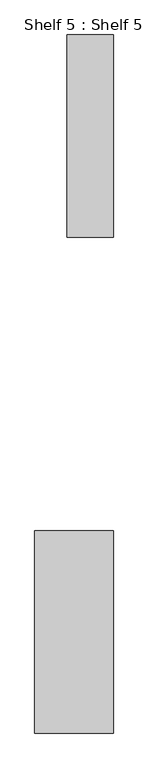
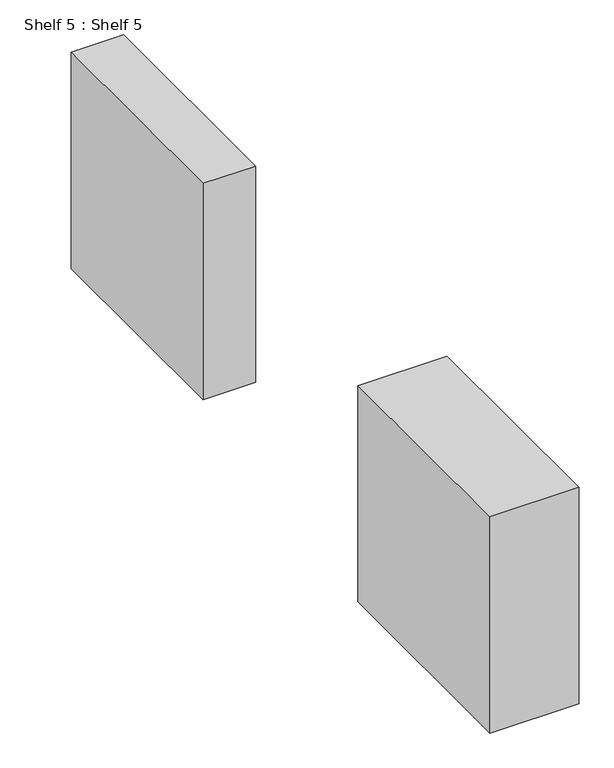
"""IFC4 building model written with IfcOpenShell, lengths in millimetres: furniture geometry, Shelf 5 : Shelf 5."""

from ifc_helpers import new_model, si_unit, origin, origin_with_axes, place, context, project, spatial, polyline, outline, extrude, source, transform, mapped, element, save


def shelf_5_shelf_5_5ccbb831(model_context):
    return source(origin(), model_context, "Body", "SweptSolid", [
        extrude(outline(polyline([(22771.8870052, 5354.3115366), (22561.5672994, 5354.3115366), (22561.5672994, 6268.7115366), (22771.8870052, 6268.7115366), (22771.8870052, 5354.3115366)])), origin_with_axes(), (0.0, 0.0, 1.0), 914.4),
        extrude(outline(polyline([(22771.8870052, 3112.7615366), (22416.2870052, 3112.7615366), (22416.2870052, 4027.1615366), (22771.8870052, 4027.1615366), (22771.8870052, 3112.7615366)])), origin_with_axes(), (0.0, 0.0, 1.0), 914.4),
    ])


if __name__ == "__main__":
    model = new_model("IFC4")
    model_context = context("Model", 3, world=origin())
    ifc_project = project(units=[si_unit("LENGTHUNIT", "METRE", prefix="MILLI")], contexts=[model_context])
    site = spatial("IfcSite", under=ifc_project)
    building = spatial("IfcBuilding", under=site)
    placement = place(None, origin())
    shelf_5_shelf_5_shape = shelf_5_shelf_5_5ccbb831(model_context)
    element("IfcFurniture", 1, ObjectType="Shelf 5 : Shelf 5", at=placement, inside=building, context=model_context, shape_type="MappedRepresentation", body=[
        mapped(shelf_5_shelf_5_shape, transform((0.0, 0.0, 0.0), x_axis=(1.0, 0.0, 0.0), y_axis=(0.0, 1.0, 0.0), z_axis=(0.0, 0.0, 1.0))),
    ])
    save(model, "model.ifc")

# Revit data of these elements
# Element 1 (IfcFurniture, "Shelf 5 : Shelf 5")
#   Materials on its faces: "food"
# Materials
#   "food": class "Glass", colour RGB 233 233 233, transparency 0, Description = "Soda Lime Glass", Cost = 0
